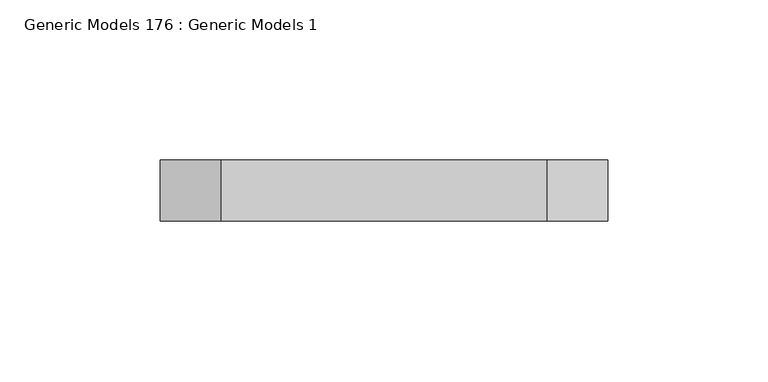
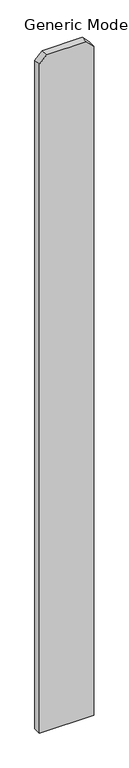
"""IFC4 building model written with IfcOpenShell, lengths in millimetres: proxy geometry, Generic Models 176 : Generic Models 1."""

from ifc_helpers import new_model, si_unit, frame, origin, place, context, project, spatial, polyline, outline, extrude, source, transform, mapped, element, save


def generic_models_176_generic_models_1_5882f369(model_context):
    return source(origin(), model_context, "Body", "SweptSolid", [
        extrude(outline(polyline([(76.2, -247981.7875), (1885.95, -247981.7875), (1905.0, -248000.8375), (1905.0, -248102.4375), (1885.95, -248121.4875), (76.2, -248121.4875), (76.2, -247981.7875)])), frame((0.0, 547.6875, 0.0), z_axis=(0.0, 1.0, 0.0), x_axis=(0.0, 0.0, 1.0)), (0.0, 0.0, 1.0), 19.05),
    ])


if __name__ == "__main__":
    model = new_model("IFC4")
    model_context = context("Model", 3, world=origin())
    ifc_project = project(units=[si_unit("LENGTHUNIT", "METRE", prefix="MILLI")], contexts=[model_context])
    site = spatial("IfcSite", under=ifc_project)
    building = spatial("IfcBuilding", under=site)
    placement = place(None, origin())
    generic_models_176_generic_models_1_shape = generic_models_176_generic_models_1_5882f369(model_context)
    element("IfcBuildingElementProxy", 1, Name="Generic Models 176 : Generic Models 1", ObjectType="Generic Models 176 : Generic Models 1", at=placement, inside=building, context=model_context, shape_type="MappedRepresentation", body=[
        mapped(generic_models_176_generic_models_1_shape, transform((0.0, 0.0, 0.0), x_axis=(1.0, 0.0, 0.0), y_axis=(0.0, 1.0, 0.0), z_axis=(0.0, 0.0, 1.0))),
    ])
    save(model, "model.ifc")

# Revit data of these elements
# Element 1 (IfcBuildingElementProxy, "Generic Models 176 : Generic Models 1")
#   Materials on its faces: "VERTICAL 1X6 CEDAR PLANKS W/ CLEAR WOOD SEALER"
# Materials
#   "VERTICAL 1X6 CEDAR PLANKS W/ CLEAR WOOD SEALER": class "Wood", colour RGB 234 198 147, transparency 0, Description = "Pinus Echinata", Cost = 0
